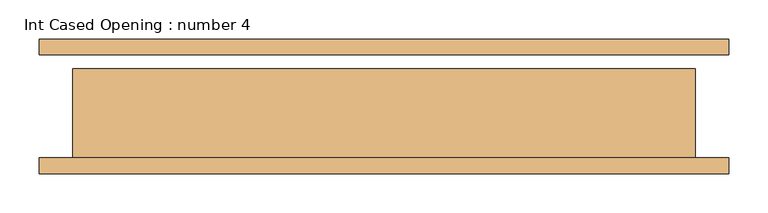
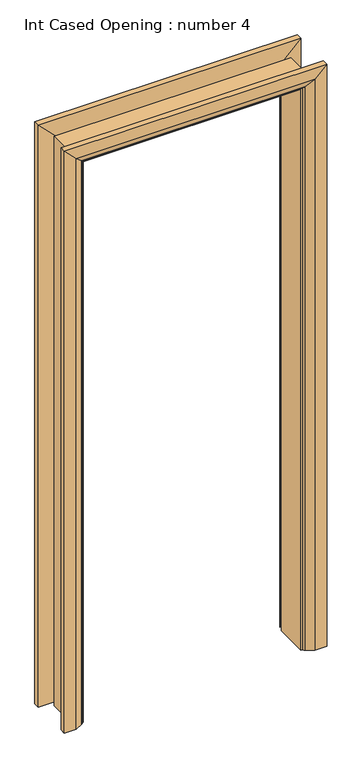
"""IFC4 building model written with IfcOpenShell, lengths in millimetres: door geometry, Int Cased Opening : number 4."""

from ifc_helpers import new_model, si_unit, frame, origin, place, context, project, spatial, circle_curve, ellipse_curve, faceted_brep, source, transform, mapped, element, save
from ifc_brep_helpers import plane_surface, cylinder_surface, advanced_brep


def int_cased_opening_number_4_3822f3ef(model_context):
    return source(origin(), model_context, "Body", "SolidModel", [
        faceted_brep([(-366.4, 57.15, 0.0), (-366.4, -57.15, 0.0), (-398.4, -57.15, 0.0), (-398.4, 57.15, 0.0), (-366.4, 57.15, 1992.0), (-366.4, -57.15, 1992.0), (-398.4, -57.15, 2024.0), (-398.4, 57.15, 2024.0), (366.4, 57.15, 0.0), (398.4, 57.15, 0.0), (398.4, -57.15, 0.0), (366.4, -57.15, 0.0), (366.4, 57.15, 1992.0), (398.4, 57.15, 2024.0), (398.4, -57.15, 2024.0), (366.4, -57.15, 1992.0)], [[[0, 1, 2, 3]], [[1, 0, 4, 5]], [[2, 1, 5, 6]], [[3, 2, 6, 7]], [[0, 3, 7, 4]], [[8, 9, 10, 11]], [[12, 13, 9, 8]], [[13, 14, 10, 9]], [[14, 15, 11, 10]], [[15, 12, 8, 11]], [[5, 4, 12, 15]], [[6, 5, 15, 14]], [[7, 6, 14, 13]], [[4, 7, 13, 12]]]),
        advanced_brep(
        [(-441.4, 95.0, 0.0), (-401.4, 95.0, 0.0), (-375.4, 81.0, 0.0), (-371.4, 75.0, 0.0), (-441.4, 75.0, 0.0), (-441.4, 95.0, 2067.0), (-401.4, 95.0, 2027.0), (-375.4, 81.0, 2001.0), (-371.4, 75.0, 1997.0), (-441.4, 75.0, 2067.0), (441.4, 95.0, 2067.0), (401.4, 95.0, 2027.0), (375.4, 81.0, 2001.0), (371.4, 75.0, 1997.0), (441.4, 75.0, 2067.0), (441.4, 95.0, 0.0), (441.4, 75.0, 0.0), (371.4, 75.0, 0.0), (375.4, 81.0, 0.0), (401.4, 95.0, 0.0)],
        [
            (0, 1),
            (1, 2),
            (2, 3, circle_curve(frame((-379.4, 74.0, 0.0), z_axis=(0.0, 0.0, -1.0), x_axis=(-1.0, 0.0, 0.0)), 8.0622577)),
            (3, 4),
            (4, 0),
            (0, 5),
            (5, 6),
            (6, 1),
            (6, 7),
            (7, 2),
            (7, 8, ellipse_curve(frame((-379.4, 74.0, 2005.0), z_axis=(-0.7071067811865475, 0.0, -0.7071067811865475), x_axis=(0.7071067811865474, 0.0, -0.7071067811865476)), 11.4017543, 8.0622577)),
            (8, 3),
            (8, 9),
            (9, 4),
            (9, 5),
            (5, 10),
            (10, 11),
            (11, 6),
            (11, 12),
            (12, 7),
            (12, 13, ellipse_curve(frame((379.4, 74.0, 2005.0), z_axis=(-0.7071067811865475, 0.0, 0.7071067811865475), x_axis=(-0.7071067811865476, 0.0, -0.7071067811865474)), 11.4017543, 8.0622577)),
            (13, 8),
            (13, 14),
            (14, 9),
            (14, 10),
            (15, 16),
            (16, 17),
            (17, 18, circle_curve(frame((379.4, 74.0, 0.0), z_axis=(0.0, 0.0, -1.0), x_axis=(1.0, 0.0, 0.0)), 8.0622577)),
            (18, 19),
            (19, 15),
            (10, 15),
            (19, 11),
            (18, 12),
            (17, 13),
            (16, 14),
        ],
        [
            plane_surface(frame((-371.4, 2.1989011, 0.0), z_axis=(0.0, 0.0, -1.0), x_axis=(1.0, 0.0, 0.0))),
            plane_surface(frame((-441.4, 95.0, 0.0), z_axis=(0.0, 1.0, 0.0), x_axis=(0.0, 0.0, 1.0))),
            plane_surface(frame((-401.4, 95.0, 0.0), z_axis=(0.4740998230350183, 0.8804710999221749, 0.0), x_axis=(0.0, 0.0, 1.0))),
            cylinder_surface(frame((-379.4, 74.0, 0.0), z_axis=(0.0, 0.0, -1.0), x_axis=(-1.0, 0.0, 0.0)), 8.0622577),
            plane_surface(frame((-371.4, 75.0, 0.0), z_axis=(0.0, -1.0, 0.0), x_axis=(0.0, 0.0, 1.0))),
            plane_surface(frame((-441.4, 75.0, 0.0), z_axis=(-1.0, 0.0, 0.0), x_axis=(0.0, 0.0, 1.0))),
            plane_surface(frame((-441.4, 95.0, 2067.0), z_axis=(0.0, 1.0, 0.0), x_axis=(1.0, 0.0, 0.0))),
            plane_surface(frame((-401.4, 95.0, 2027.0), z_axis=(0.0, 0.8804710999221749, -0.4740998230350183), x_axis=(1.0, 0.0, 0.0))),
            cylinder_surface(frame((-371.4, 74.0, 2005.0), z_axis=(-1.0, 0.0, 0.0), x_axis=(0.0, 0.0, 1.0)), 8.0622577),
            plane_surface(frame((-371.4, 75.0, 1997.0), z_axis=(0.0, -1.0, 0.0), x_axis=(1.0, 0.0, 0.0))),
            plane_surface(frame((-441.4, 75.0, 2067.0), z_axis=(0.0, 0.0, 1.0), x_axis=(1.0, 0.0, 0.0))),
            plane_surface(frame((371.4, 2.1989011, 0.0), z_axis=(0.0, 0.0, -1.0), x_axis=(-1.0, 0.0, 0.0))),
            plane_surface(frame((441.4, 95.0, 2067.0), z_axis=(0.0, 1.0, 0.0), x_axis=(0.0, 0.0, -1.0))),
            plane_surface(frame((401.4, 95.0, 2027.0), z_axis=(-0.4740998230350183, 0.8804710999221749, 0.0), x_axis=(0.0, 0.0, -1.0))),
            cylinder_surface(frame((379.4, 74.0, 1997.0), z_axis=(0.0, 0.0, 1.0), x_axis=(1.0, 0.0, 0.0)), 8.0622577),
            plane_surface(frame((371.4, 75.0, 1997.0), z_axis=(0.0, -1.0, 0.0), x_axis=(0.0, 0.0, -1.0))),
            plane_surface(frame((441.4, 75.0, 2067.0), z_axis=(1.0, 0.0, 0.0), x_axis=(0.0, 0.0, -1.0))),
        ],
        [
            (0, [[1, 2, 3, 4, 5]]),
            (1, [[-1, 6, 7, 8]]),
            (2, [[-2, -8, 9, 10]]),
            (3, [[-3, -10, 11, 12]]),
            (4, [[-4, -12, 13, 14]]),
            (5, [[-5, -14, 15, -6]]),
            (6, [[-7, 16, 17, 18]]),
            (7, [[-9, -18, 19, 20]]),
            (8, [[-11, -20, 21, 22]]),
            (9, [[-13, -22, 23, 24]]),
            (10, [[-15, -24, 25, -16]]),
            (11, [[26, 27, 28, 29, 30]]),
            (12, [[-17, 31, -30, 32]]),
            (13, [[-19, -32, -29, 33]]),
            (14, [[-21, -33, -28, 34]]),
            (15, [[-23, -34, -27, 35]]),
            (16, [[-25, -35, -26, -31]]),
        ],
    ),
        advanced_brep(
        [(-441.4, -77.15, 0.0), (-441.4, -57.15, 0.0), (-371.4, -57.15, 0.0), (-375.4, -63.15, 0.0), (-401.4, -77.15, 0.0), (-441.4, -77.15, 2067.0), (-441.4, -57.15, 2067.0), (-371.4, -57.15, 1997.0), (-375.4, -63.15, 2001.0), (-401.4, -77.15, 2027.0), (441.4, -77.15, 2067.0), (441.4, -57.15, 2067.0), (371.4, -57.15, 1997.0), (375.4, -63.15, 2001.0), (401.4, -77.15, 2027.0), (441.4, -77.15, 0.0), (401.4, -77.15, 0.0), (375.4, -63.15, 0.0), (371.4, -57.15, 0.0), (441.4, -57.15, 0.0)],
        [
            (0, 1),
            (1, 2),
            (2, 3, circle_curve(frame((-379.4, -56.15, 0.0), z_axis=(0.0, 0.0, -1.0), x_axis=(-1.0, 0.0, 0.0)), 8.0622577)),
            (3, 4),
            (4, 0),
            (0, 5),
            (5, 6),
            (6, 1),
            (6, 7),
            (7, 2),
            (7, 8, ellipse_curve(frame((-379.4, -56.15, 2005.0), z_axis=(-0.7071067811865475, 0.0, -0.7071067811865475), x_axis=(0.7071067811865474, 0.0, -0.7071067811865476)), 11.4017543, 8.0622577)),
            (8, 3),
            (8, 9),
            (9, 4),
            (9, 5),
            (5, 10),
            (10, 11),
            (11, 6),
            (11, 12),
            (12, 7),
            (12, 13, ellipse_curve(frame((379.4, -56.15, 2005.0), z_axis=(-0.7071067811865475, 0.0, 0.7071067811865475), x_axis=(-0.7071067811865476, 0.0, -0.7071067811865474)), 11.4017543, 8.0622577)),
            (13, 8),
            (13, 14),
            (14, 9),
            (14, 10),
            (15, 16),
            (16, 17),
            (17, 18, circle_curve(frame((379.4, -56.15, 0.0), z_axis=(0.0, 0.0, -1.0), x_axis=(1.0, 0.0, 0.0)), 8.0622577)),
            (18, 19),
            (19, 15),
            (10, 15),
            (19, 11),
            (18, 12),
            (17, 13),
            (16, 14),
        ],
        [
            plane_surface(frame((-371.4, -129.9510989, 0.0), z_axis=(0.0, 0.0, -1.0), x_axis=(1.0, 0.0, 0.0))),
            plane_surface(frame((-441.4, -77.15, 0.0), z_axis=(-1.0, 0.0, 0.0), x_axis=(0.0, 0.0, 1.0))),
            plane_surface(frame((-441.4, -57.15, 0.0), z_axis=(0.0, 1.0, 0.0), x_axis=(0.0, 0.0, 1.0))),
            cylinder_surface(frame((-379.4, -56.15, 0.0), z_axis=(0.0, 0.0, -1.0), x_axis=(-1.0, 0.0, 0.0)), 8.0622577),
            plane_surface(frame((-375.4, -63.15, 0.0), z_axis=(0.4740998230350183, -0.8804710999221749, 0.0), x_axis=(0.0, 0.0, 1.0))),
            plane_surface(frame((-401.4, -77.15, 0.0), z_axis=(0.0, -1.0, 0.0), x_axis=(0.0, 0.0, 1.0))),
            plane_surface(frame((-441.4, -77.15, 2067.0), z_axis=(0.0, 0.0, 1.0), x_axis=(1.0, 0.0, 0.0))),
            plane_surface(frame((-441.4, -57.15, 2067.0), z_axis=(0.0, 1.0, 0.0), x_axis=(1.0, 0.0, 0.0))),
            cylinder_surface(frame((-371.4, -56.15, 2005.0), z_axis=(-1.0, 0.0, 0.0), x_axis=(0.0, 0.0, 1.0)), 8.0622577),
            plane_surface(frame((-375.4, -63.15, 2001.0), z_axis=(0.0, -0.8804710999221749, -0.4740998230350183), x_axis=(1.0, 0.0, 0.0))),
            plane_surface(frame((-401.4, -77.15, 2027.0), z_axis=(0.0, -1.0, 0.0), x_axis=(1.0, 0.0, 0.0))),
            plane_surface(frame((371.4, -129.9510989, 0.0), z_axis=(0.0, 0.0, -1.0), x_axis=(-1.0, 0.0, 0.0))),
            plane_surface(frame((441.4, -77.15, 2067.0), z_axis=(1.0, 0.0, 0.0), x_axis=(0.0, 0.0, -1.0))),
            plane_surface(frame((441.4, -57.15, 2067.0), z_axis=(0.0, 1.0, 0.0), x_axis=(0.0, 0.0, -1.0))),
            cylinder_surface(frame((379.4, -56.15, 1997.0), z_axis=(0.0, 0.0, 1.0), x_axis=(1.0, 0.0, 0.0)), 8.0622577),
            plane_surface(frame((375.4, -63.15, 2001.0), z_axis=(-0.4740998230350183, -0.8804710999221749, 0.0), x_axis=(0.0, 0.0, -1.0))),
            plane_surface(frame((401.4, -77.15, 2027.0), z_axis=(0.0, -1.0, 0.0), x_axis=(0.0, 0.0, -1.0))),
        ],
        [
            (0, [[1, 2, 3, 4, 5]]),
            (1, [[-1, 6, 7, 8]]),
            (2, [[-2, -8, 9, 10]]),
            (3, [[-3, -10, 11, 12]]),
            (4, [[-4, -12, 13, 14]]),
            (5, [[-5, -14, 15, -6]]),
            (6, [[-7, 16, 17, 18]]),
            (7, [[-9, -18, 19, 20]]),
            (8, [[-11, -20, 21, 22]]),
            (9, [[-13, -22, 23, 24]]),
            (10, [[-15, -24, 25, -16]]),
            (11, [[26, 27, 28, 29, 30]]),
            (12, [[-17, 31, -30, 32]]),
            (13, [[-19, -32, -29, 33]]),
            (14, [[-21, -33, -28, 34]]),
            (15, [[-23, -34, -27, 35]]),
            (16, [[-25, -35, -26, -31]]),
        ],
    ),
    ])


if __name__ == "__main__":
    model = new_model("IFC4")
    model_context = context("Model", 3, world=origin())
    ifc_project = project(units=[si_unit("LENGTHUNIT", "METRE", prefix="MILLI")], contexts=[model_context])
    site = spatial("IfcSite", under=ifc_project)
    building = spatial("IfcBuilding", under=site)
    placement = place(None, origin())
    int_cased_opening_number_4_shape = int_cased_opening_number_4_3822f3ef(model_context)
    element("IfcDoor", 1, ObjectType="Int Cased Opening : number 4", at=placement, inside=building, context=model_context, shape_type="MappedRepresentation", body=[
        mapped(int_cased_opening_number_4_shape, transform((0.0, 0.0, 0.0), x_axis=(1.0, 0.0, 0.0), y_axis=(0.0, 1.0, 0.0), z_axis=(0.0, 0.0, 1.0))),
    ])
    save(model, "model.ifc")

# Revit data of these elements
# Type "Int Cased Opening : number 4"
#   Type Mark = "104"
#   Operation = "UserDefined"
#   Manufacturer = "Revit"
#   Keynote = "L20"
#   Width = 2' - 8"
#   Rough Width = 2' - 8"
#   Rough Height = 6' - 8"
#   Height = 6' - 8"
#   Frame Thickness = 0' - 1.25984"
#   Architrave Setback = 0' - 0.19685"
#   Vis - Architrave = yes
#   Material Frame = Door - Frame/Mullion
#   Material Architrave = Door - Architrave
#   Function = (empty or 0)
#   Wall Closure = (empty or 0)
# Element 1 (IfcDoor, "Int Cased Opening : number 4")
#   Materials on its faces: "Door - Architrave", "Door - Frame/Mullion"
# Materials
#   "Door - Frame/Mullion": class "Wood", colour RGB 212 179 113, transparency 0, Keynote = "L20", Cost = 0
#   "Door - Architrave": class "Wood", colour RGB 192 192 192, transparency 0, Keynote = "P20", Cost = 0
